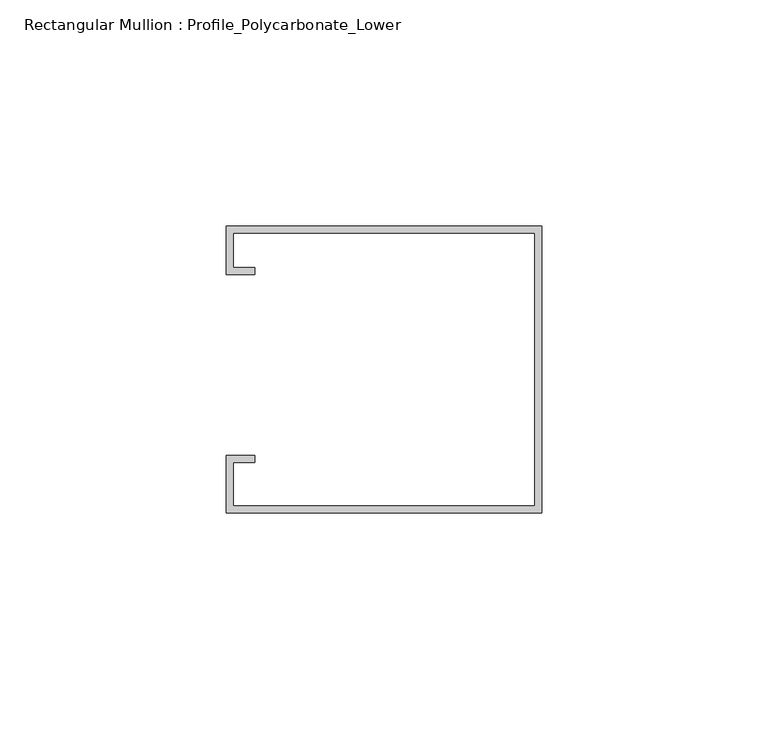
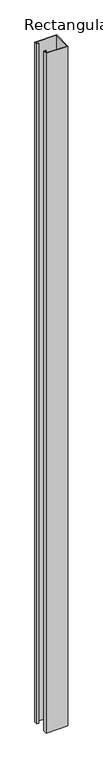
"""IFC4 building model written with IfcOpenShell, lengths in millimetres: member geometry, Rectangular Mullion : Profile_Polycarbonate_Lower."""

from ifc_helpers import new_model, si_unit, frame, origin, place, context, project, spatial, polyline, outline, extrude, source, transform, mapped, element, save


def rectangular_mullion_profile_polycarbonate_lower_76a3051d(model_context):
    return source(origin(), model_context, "Body", "SweptSolid", [
        extrude(outline(polyline([(0.0, -32.7), (-69.85, -32.7), (-69.85, -20.0), (-63.5, -20.0), (-63.5, -21.5875), (-68.2625, -21.5875), (-68.2625, -31.1125), (-1.5875, -31.1125), (-1.5875, 29.2125), (-68.2625, 29.2125), (-68.2625, 21.5875), (-63.5, 21.5875), (-63.5, 20.0), (-69.85, 20.0), (-69.85, 30.8), (0.0, 30.8), (0.0, -32.7)])), frame((0.0, 0.0, -2319.967633), z_axis=(0.0, 0.0, 1.0), x_axis=(1.0, 0.0, 0.0)), (0.0, 0.0, 1.0), 2319.967633),
    ])


if __name__ == "__main__":
    model = new_model("IFC4")
    model_context = context("Model", 3, world=origin())
    ifc_project = project(units=[si_unit("LENGTHUNIT", "METRE", prefix="MILLI")], contexts=[model_context])
    site = spatial("IfcSite", under=ifc_project)
    building = spatial("IfcBuilding", under=site)
    placement = place(None, origin())
    rectangular_mullion_profile_polycarbonate_lower_shape = rectangular_mullion_profile_polycarbonate_lower_76a3051d(model_context)
    element("IfcMember", 1, ObjectType="Rectangular Mullion : Profile_Polycarbonate_Lower", at=placement, inside=building, context=model_context, shape_type="MappedRepresentation", body=[
        mapped(rectangular_mullion_profile_polycarbonate_lower_shape, transform((0.0, 0.0, 0.0), x_axis=(1.0, 0.0, 0.0), y_axis=(0.0, 1.0, 0.0), z_axis=(0.0, 0.0, 1.0))),
    ])
    save(model, "model.ifc")

# Revit data of these elements
# Type "Rectangular Mullion : Profile_Polycarbonate_Lower"
#   built-in parameter 1007322 = 0.208333 (stored number, unit not read)
#   built-in parameter 1007321 = 0 (stored number, unit not read)
#   built-in parameter 1007320 = 0.00520833 (stored number, unit not read)
# Element 1 (IfcMember, "Rectangular Mullion : Profile_Polycarbonate_Lower")
#   Materials on its faces: "ALUMINUM PROFILE AT POLYCARBONATE PANEL"
# Materials
#   "ALUMINUM PROFILE AT POLYCARBONATE PANEL": class "Metal", colour RGB 244 244 244, transparency 0, Description = "Aluminum 6061", Cost = 0
